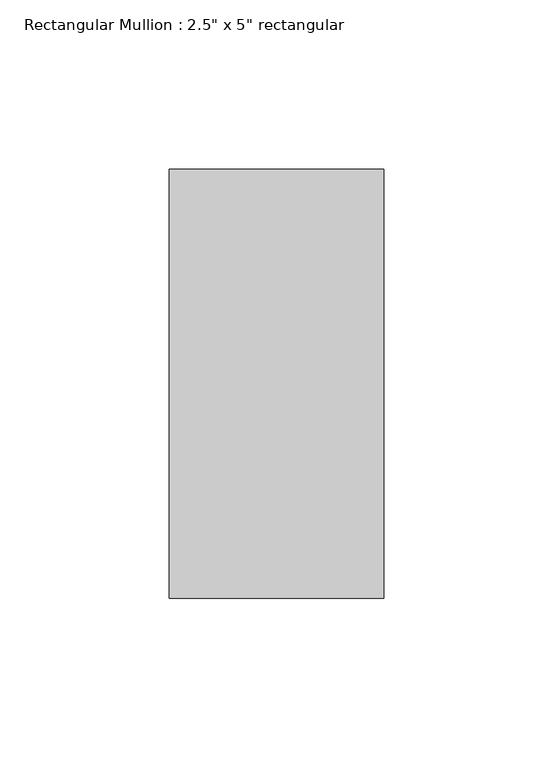
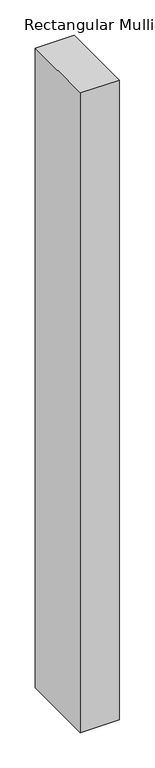
"""IFC4 building model written with IfcOpenShell, lengths in millimetres: member geometry."""

from ifc_helpers import new_model, si_unit, frame, origin, place, context, project, spatial, polyline, outline, extrude, source, transform, mapped, element, save


def member_1f6f54fd(model_context):
    return source(origin(), model_context, "Body", "SweptSolid", [
        extrude(outline(polyline([(0.0, 63.5), (0.0, -63.5), (-63.5, -63.5), (-63.5, 63.5), (0.0, 63.5)])), frame((0.0, 0.0, -1103.9315359), z_axis=(0.0, 0.0, 1.0), x_axis=(1.0, 0.0, 0.0)), (0.0, 0.0, 1.0), 1103.9315359),
    ])


if __name__ == "__main__":
    model = new_model("IFC4")
    model_context = context("Model", 3, world=origin())
    ifc_project = project(units=[si_unit("LENGTHUNIT", "METRE", prefix="MILLI")], contexts=[model_context])
    site = spatial("IfcSite", under=ifc_project)
    building = spatial("IfcBuilding", under=site)
    placement = place(None, origin())
    member_shape = member_1f6f54fd(model_context)
    element("IfcMember", 1, ObjectType="Rectangular Mullion : 2.5\" x 5\" rectangular", at=placement, inside=building, context=model_context, shape_type="MappedRepresentation", body=[
        mapped(member_shape, transform((0.0, 0.0, 0.0), x_axis=(1.0, 0.0, 0.0), y_axis=(0.0, 1.0, 0.0), z_axis=(0.0, 0.0, 1.0))),
    ])
    save(model, "model.ifc")

# Revit data of these elements
# Type "Rectangular Mullion : 2.5\" x 5\" rectangular"
#   built-in parameter 1007304 = 0.416667 (stored number, unit not read)
#   built-in parameter 1007301 = 0.104167 (stored number, unit not read)
#   built-in parameter 1007300 = 0.104167 (stored number, unit not read)
# Element 1 (IfcMember, "Rectangular Mullion : 2.5\" x 5\" rectangular")
#   Materials on its faces: "Aluminum"
# Materials
#   "Aluminum": class "Metal", colour RGB 247 247 247, transparency 0, Description = "Aluminum 6061", Cost = 0
